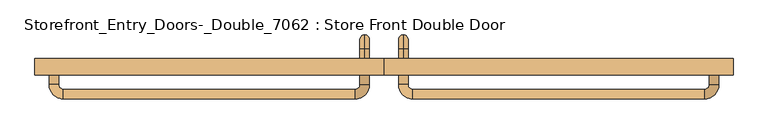
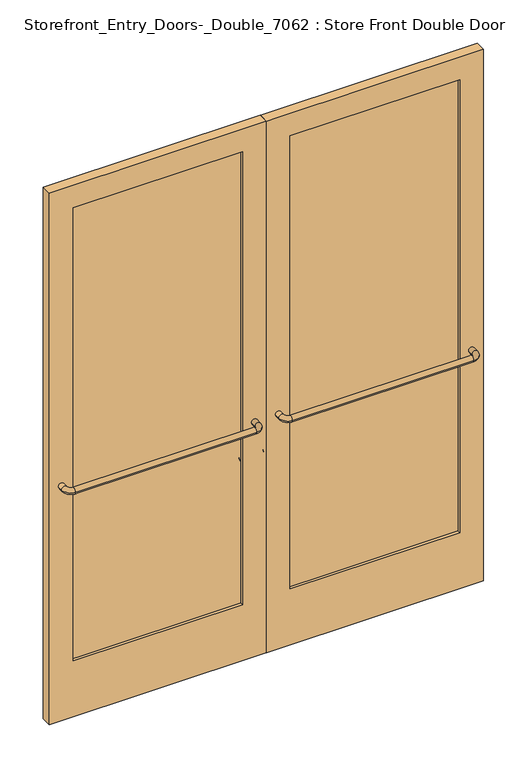
"""IFC4 building model written with IfcOpenShell, lengths in millimetres: door geometry, Storefront_Entry_Doors-_Double_7062 : Store Front Double Door."""

import ifcopenshell
import ifcopenshell.guid

model = None  # the IFC model being written
_history = None  # IfcOwnerHistory: only IFC2X3 demands one
_inside = {}  # id of a spatial element -> (the spatial element, [elements in it])
_under = {}  # id of a project, library or spatial element -> (it, [spatial elements below it])
_declared = {}  # id of a project -> (the project, [libraries it declares])
_typed = {}  # id of a type object -> (the type object, [elements of that type])
_made_of = {}  # id of a material, layer set ... -> (it, [elements and type objects made of it])


def new_model(schema):
    """Start an empty IFC model of exactly this schema.

    Asked for "IFC4X3", IfcOpenShell would pick the latest addendum, in which some entities
    have other attributes; the version numbers below select the first issue.
    IFC2X3 requires an IfcOwnerHistory on every rooted entity: one is made here for all.
    """
    global model, _history
    if schema == "IFC4X3":
        model = ifcopenshell.file(schema_version=(4, 3, 0, 0))
    else:
        model = ifcopenshell.file(schema=schema)
    _inside.clear()
    _under.clear()
    _declared.clear()
    _typed.clear()
    _made_of.clear()
    _history = None
    if model.schema == "IFC2X3":
        org = make("IfcOrganization", Name="unknown")
        user = make(
            "IfcPersonAndOrganization",
            ThePerson=make("IfcPerson", FamilyName="unknown"),
            TheOrganization=org,
        )
        app = make(
            "IfcApplication",
            ApplicationDeveloper=org,
            Version="unknown",
            ApplicationFullName="unknown",
            ApplicationIdentifier="unknown",
        )
        _history = make(
            "IfcOwnerHistory",
            OwningUser=user,
            OwningApplication=app,
            ChangeAction="ADDED",
            CreationDate=0,
        )
    return model


def make(cls, **values):
    """One entity of the class cls with the attributes given. An attribute that is None is left unset."""
    return model.create_entity(
        cls, **{name: value for name, value in values.items() if value is not None}
    )


def rooted(cls, **values):
    """An entity with a GlobalId (a new one), such as an element, a storey or a relation."""
    return make(cls, GlobalId=ifcopenshell.guid.new(), OwnerHistory=_history, **values)


def si_unit(unit_type, name, prefix=None):
    """IfcSIUnit, for example si_unit("LENGTHUNIT", "METRE", prefix="MILLI")."""
    return make("IfcSIUnit", UnitType=unit_type, Prefix=prefix, Name=name)


def assignment(units):
    """IfcUnitAssignment: the units of a project."""
    return None if units is None else make("IfcUnitAssignment", Units=units)


def point(xyz):
    """IfcCartesianPoint."""
    return None if xyz is None else make("IfcCartesianPoint", Coordinates=xyz)


def direction(xyz):
    """IfcDirection."""
    return None if xyz is None else make("IfcDirection", DirectionRatios=xyz)


def frame(location, z_axis=None, x_axis=None):
    """IfcAxis2Placement3D, a coordinate frame: its origin and axes. An axis left out is left unset."""
    return make(
        "IfcAxis2Placement3D",
        Location=point(location),
        Axis=direction(z_axis),
        RefDirection=direction(x_axis),
    )


def origin():
    """The frame at (0, 0, 0) with its axes left unset."""
    return frame((0.0, 0.0, 0.0))


def place(relative_to, where):
    """IfcLocalPlacement: puts the frame where relative to a parent placement (None: the world)."""
    return make(
        "IfcLocalPlacement", PlacementRelTo=relative_to, RelativePlacement=where
    )


def context(
    kind, dimensions, precision=None, world=None, true_north=None, identifier=None
):
    """IfcGeometricRepresentationContext, for example the 3D "Model" context."""
    return make(
        "IfcGeometricRepresentationContext",
        ContextIdentifier=identifier,
        ContextType=kind,
        CoordinateSpaceDimension=dimensions,
        Precision=precision,
        WorldCoordinateSystem=world,
        TrueNorth=true_north,
    )


def project(units=None, contexts=None):
    """IfcProject with its units and contexts."""
    return rooted(
        "IfcProject",
        Name="project",
        RepresentationContexts=contexts,
        UnitsInContext=assignment(units),
    )


def spatial(cls, under=None, at=None, **own):
    """A site, building, storey or space (cls), placed at a placement, below another one or the project."""
    s = rooted(cls, ObjectPlacement=at, **own)
    if under is not None:
        _under.setdefault(under.id(), (under, []))[1].append(s)
    return s


def polyline(points):
    """IfcPolyline through the points."""
    return make("IfcPolyline", Points=[point(p) for p in points])


def circle_curve(where, radius):
    """IfcCircle in the frame where."""
    return make("IfcCircle", Position=where, Radius=radius)


def ellipse_curve(where, semi_axis1, semi_axis2):
    """IfcEllipse in the frame where."""
    return make(
        "IfcEllipse", Position=where, SemiAxis1=semi_axis1, SemiAxis2=semi_axis2
    )


def trimmed(basis, trim1, trim2, sense, master):
    """IfcTrimmedCurve: the piece of a basis curve between two trims."""
    return make(
        "IfcTrimmedCurve",
        BasisCurve=basis,
        Trim1=trim1,
        Trim2=trim2,
        SenseAgreement=sense,
        MasterRepresentation=master,
    )


def outline(outer, holes=None, kind="AREA"):
    """IfcArbitraryClosedProfileDef: a profile drawn as a closed curve; with holes, ...WithVoids."""
    if holes is None:
        return make("IfcArbitraryClosedProfileDef", ProfileType=kind, OuterCurve=outer)
    return make(
        "IfcArbitraryProfileDefWithVoids",
        ProfileType=kind,
        OuterCurve=outer,
        InnerCurves=holes,
    )


def extrude(swept, where, along, depth):
    """IfcExtrudedAreaSolid: the profile swept, set in the frame where, extruded along a direction by depth."""
    return make(
        "IfcExtrudedAreaSolid",
        SweptArea=swept,
        Position=where,
        ExtrudedDirection=direction(along),
        Depth=depth,
    )


def shape(context_of_items, identifier, shape_type, items):
    """IfcShapeRepresentation: the items that make up one representation, for example the "Body"."""
    return make(
        "IfcShapeRepresentation",
        ContextOfItems=context_of_items,
        RepresentationIdentifier=identifier,
        RepresentationType=shape_type,
        Items=items,
    )


def source(mapping_origin, context_of_items, identifier, shape_type, items):
    """IfcRepresentationMap: a shape defined once, which mapped items show again and again."""
    return make(
        "IfcRepresentationMap",
        MappingOrigin=mapping_origin,
        MappedRepresentation=shape(context_of_items, identifier, shape_type, items),
    )


def transform(
    local_origin,
    x_axis=None,
    y_axis=None,
    z_axis=None,
    scale=None,
    scale2=None,
    scale3=None,
    uniform=True,
):
    """IfcCartesianTransformationOperator3D, or its non-uniform kind. x_axis, y_axis, z_axis: its Axis1, 2, 3."""
    if uniform:
        return make(
            "IfcCartesianTransformationOperator3D",
            Axis1=direction(x_axis),
            Axis2=direction(y_axis),
            LocalOrigin=point(local_origin),
            Scale=scale,
            Axis3=direction(z_axis),
        )
    return make(
        "IfcCartesianTransformationOperator3DnonUniform",
        Axis1=direction(x_axis),
        Axis2=direction(y_axis),
        LocalOrigin=point(local_origin),
        Scale=scale,
        Axis3=direction(z_axis),
        Scale2=scale2,
        Scale3=scale3,
    )


def mapped(mapping_source, mapping_target):
    """IfcMappedItem: shows the shape of a source again, moved by a transform."""
    return make(
        "IfcMappedItem", MappingSource=mapping_source, MappingTarget=mapping_target
    )


def made_of(thing, what):
    """Note that an element or type object is made of a material, layer set ...; save() writes the relation."""
    if what is not None:
        _made_of.setdefault(what.id(), (what, []))[1].append(thing)
    return thing


def element(
    cls,
    number,
    at=None,
    inside=None,
    cuts=None,
    type_object=None,
    material=None,
    context=None,
    identifier="Body",
    shape_type=None,
    held_by="IfcProductDefinitionShape",
    body=None,
    shapes=None,
    **own,
):
    """One element of the class cls, such as IfcWall. Its Tag is "e" and its number.

    at: its placement. inside: the storey or other place that contains it. cuts: it is an
    opening in that element (IfcRelVoidsElement). A single representation is given by context,
    identifier, shape_type and body (its items); several are given by shapes. held_by: the class
    of the entity that holds the representations. save() writes the other relations.
    """
    e = rooted(cls, Tag="e%d" % number, ObjectPlacement=at, **own)
    if body is not None:
        shapes = [shape(context, identifier, shape_type, body)]
    if shapes is not None:
        e.Representation = make(held_by, Representations=shapes)
    if inside is not None:
        _inside.setdefault(inside.id(), (inside, []))[1].append(e)
    if cuts is not None:
        rooted(
            "IfcRelVoidsElement", RelatingBuildingElement=cuts, RelatedOpeningElement=e
        )
    if type_object is not None:
        _typed.setdefault(type_object.id(), (type_object, []))[1].append(e)
    return made_of(e, material)


def aggregate(whole, parts):
    """IfcRelAggregates: a whole, such as a stair, and the parts it consists of."""
    return rooted("IfcRelAggregates", RelatingObject=whole, RelatedObjects=parts)


def save(model, path):
    """Write the relations noted so far, then the file.

    IfcRelAggregates (storeys below a building ...), IfcRelContainedInSpatialStructure (elements
    in a storey), IfcRelDefinesByType, IfcRelAssociatesMaterial and IfcRelDeclares: one each for
    every whole, place, type object, material and project.
    """
    for whole, parts in _under.values():
        aggregate(whole, parts)
    for where, things in _inside.values():
        rooted(
            "IfcRelContainedInSpatialStructure",
            RelatedElements=things,
            RelatingStructure=where,
        )
    for kind, things in _typed.values():
        rooted("IfcRelDefinesByType", RelatedObjects=things, RelatingType=kind)
    for what, things in _made_of.values():
        rooted("IfcRelAssociatesMaterial", RelatedObjects=things, RelatingMaterial=what)
    for by, libraries in _declared.values():
        rooted("IfcRelDeclares", RelatingContext=by, RelatedDefinitions=libraries)
    model.write(path)


def plane_surface(at):
    """IfcPlane: the flat surface through the origin of the frame at, square to its z axis."""
    return make("IfcPlane", Position=at)


def cylinder_surface(at, radius):
    """IfcCylindricalSurface: all points at the distance radius from the z axis of the frame at."""
    return make("IfcCylindricalSurface", Position=at, Radius=radius)


def revolved_surface(curve, axis_point, axis_direction):
    """IfcSurfaceOfRevolution: the curve turned about the line through axis_point along axis_direction."""
    return make(
        "IfcSurfaceOfRevolution",
        SweptCurve=make("IfcArbitraryOpenProfileDef", ProfileType="CURVE", Curve=curve),
        AxisPosition=make("IfcAxis1Placement", Location=point(axis_point), Axis=direction(axis_direction)),
    )


def advanced_brep(points, edges, surfaces, faces):
    """IfcAdvancedBrep: a solid bounded by faces that lie on surfaces and meet in shared edges.

    An edge is (start, end): straight between two places in points (the first is 0);
    or (start, end, curve); or (start, end, curve, False) where it runs against its curve.
    A face is (place in surfaces, loops), or (place, loops, False) where it looks against
    its surface's normal. A loop lists edges by number (the first is 1), with a minus sign
    where the edge is run from its end to its start. The first loop is the outer one.
    """
    corners = [point(p) for p in points]
    vertices = [make("IfcVertexPoint", VertexGeometry=c) for c in corners]
    made = []
    for start, end, *more in edges:
        made.append(
            make(
                "IfcEdgeCurve",
                EdgeStart=vertices[start],
                EdgeEnd=vertices[end],
                EdgeGeometry=more[0] if more else make("IfcPolyline", Points=[corners[start], corners[end]]),
                SameSense=more[1] if len(more) > 1 else True,
            )
        )
    hull = []
    for where, loops, *sense in faces:
        bounds = []
        for j, loop in enumerate(loops):
            ring = [make("IfcOrientedEdge", EdgeElement=made[abs(k) - 1], Orientation=k > 0) for k in loop]
            bounds.append(
                make(
                    "IfcFaceOuterBound" if j == 0 else "IfcFaceBound",
                    Bound=make("IfcEdgeLoop", EdgeList=ring),
                    Orientation=True,
                )
            )
        hull.append(make("IfcAdvancedFace", Bounds=bounds, FaceSurface=surfaces[where], SameSense=sense[0] if sense else True))
    return make("IfcAdvancedBrep", Outer=make("IfcClosedShell", CfsFaces=hull))


def storefront_entry_doors_double_7062_store_front_double_door_b38478ba(model_context):
    return source(origin(), model_context, "Body", "SolidModel", [
        advanced_brep(
        [(51.59375, 50.8, 1079.5), (51.59375, 50.8, 1054.1), (51.59375, 76.2, 1079.5), (51.59375, 76.2, 1054.1), (51.59375, 88.9, 1041.4), (51.59375, 114.3, 1041.4), (51.59375, 114.3, 863.6), (51.59375, 88.9, 863.6), (51.59375, 76.2, 850.9), (51.59375, 76.2, 825.5), (51.59375, 50.8, 825.5), (51.59375, 50.8, 850.9)],
        [
            (0, 1, circle_curve(frame((51.59375, 50.8, 1066.8), z_axis=(0.0, -1.0, 0.0), x_axis=(0.0, 0.0, -1.0)), 12.7)),
            (1, 0, circle_curve(frame((51.59375, 50.8, 1066.8), z_axis=(0.0, -1.0, 0.0), x_axis=(0.0, 0.0, -1.0)), 12.7)),
            (0, 2),
            (2, 3, circle_curve(frame((51.59375, 76.2, 1066.8), z_axis=(0.0, -1.0, 0.0), x_axis=(0.0, 0.0, -1.0)), 12.7)),
            (3, 1),
            (3, 2, circle_curve(frame((51.59375, 76.2, 1066.8), z_axis=(0.0, -1.0, 0.0), x_axis=(0.0, 0.0, -1.0)), 12.7)),
            (4, 3, circle_curve(frame((51.59375, 76.2, 1041.4), z_axis=(1.0, 0.0, 0.0), x_axis=(0.0, 0.0, 1.0)), 12.7)),
            (2, 5, circle_curve(frame((51.59375, 76.2, 1041.4), z_axis=(-1.0, 0.0, 0.0), x_axis=(0.0, 0.0, 1.0)), 38.1)),
            (5, 4, circle_curve(frame((51.59375, 101.6, 1041.4), z_axis=(0.0, 0.0, 1.0), x_axis=(0.0, -1.0, 0.0)), 12.7)),
            (4, 5, circle_curve(frame((51.59375, 101.6, 1041.4), z_axis=(0.0, 0.0, 1.0), x_axis=(0.0, -1.0, 0.0)), 12.7)),
            (5, 6),
            (6, 7, circle_curve(frame((51.59375, 101.6, 863.6), z_axis=(0.0, 0.0, 1.0), x_axis=(0.0, -1.0, 0.0)), 12.7)),
            (7, 4),
            (7, 6, circle_curve(frame((51.59375, 101.6, 863.6), z_axis=(0.0, 0.0, 1.0), x_axis=(0.0, -1.0, 0.0)), 12.7)),
            (8, 7, circle_curve(frame((51.59375, 76.2, 863.6), z_axis=(1.0, 0.0, 0.0), x_axis=(0.0, 1.0, 0.0)), 12.7)),
            (6, 9, circle_curve(frame((51.59375, 76.2, 863.6), z_axis=(-1.0, 0.0, 0.0), x_axis=(0.0, 1.0, 0.0)), 38.1)),
            (9, 8, circle_curve(frame((51.59375, 76.2, 838.2), z_axis=(0.0, 1.0, 0.0), x_axis=(0.0, 0.0, 1.0)), 12.7)),
            (8, 9, circle_curve(frame((51.59375, 76.2, 838.2), z_axis=(0.0, 1.0, 0.0), x_axis=(0.0, 0.0, 1.0)), 12.7)),
            (10, 11, circle_curve(frame((51.59375, 50.8, 838.2), z_axis=(0.0, -1.0, 0.0), x_axis=(0.0, 0.0, 1.0)), 12.7)),
            (11, 10, circle_curve(frame((51.59375, 50.8, 838.2), z_axis=(0.0, -1.0, 0.0), x_axis=(0.0, 0.0, 1.0)), 12.7)),
            (9, 10),
            (11, 8),
        ],
        [
            plane_surface(frame((51.59375, 50.8, 1066.8), z_axis=(0.0, -1.0, 0.0), x_axis=(-1.0, 0.0, 0.0))),
            cylinder_surface(frame((51.59375, 50.8, 1066.8), z_axis=(0.0, -1.0, 0.0), x_axis=(0.0, 0.0, -1.0)), 12.7),
            revolved_surface(trimmed(ellipse_curve(frame((51.59375, 76.2, 1066.8), z_axis=(0.0, -1.0, 0.0), x_axis=(0.0, 0.0, -1.0)), 12.7, 12.7), [point((51.59375, 76.2, 1079.5))], [point((51.59375, 76.2, 1054.1))], True, "CARTESIAN"), (51.59375, 76.2, 1041.4), (-1.0, 0.0, 0.0)),
            revolved_surface(trimmed(ellipse_curve(frame((51.59375, 76.2, 1066.8), z_axis=(0.0, -1.0, 0.0), x_axis=(0.0, 0.0, -1.0)), 12.7, 12.7), [point((51.59375, 76.2, 1054.1))], [point((51.59375, 76.2, 1079.5))], True, "CARTESIAN"), (51.59375, 76.2, 1041.4), (-1.0, 0.0, 0.0)),
            cylinder_surface(frame((51.59375, 101.6, 1041.4), z_axis=(0.0, 0.0, 1.0), x_axis=(0.0, -1.0, 0.0)), 12.7),
            revolved_surface(trimmed(ellipse_curve(frame((51.59375, 101.6, 863.6), z_axis=(0.0, 0.0, 1.0), x_axis=(0.0, -1.0, 0.0)), 12.7, 12.7), [point((51.59375, 114.3, 863.6))], [point((51.59375, 88.9, 863.6))], True, "CARTESIAN"), (51.59375, 76.2, 863.6), (-1.0, 0.0, 0.0)),
            revolved_surface(trimmed(ellipse_curve(frame((51.59375, 101.6, 863.6), z_axis=(0.0, 0.0, 1.0), x_axis=(0.0, -1.0, 0.0)), 12.7, 12.7), [point((51.59375, 88.9, 863.6))], [point((51.59375, 114.3, 863.6))], True, "CARTESIAN"), (51.59375, 76.2, 863.6), (-1.0, 0.0, 0.0)),
            plane_surface(frame((51.59375, 50.8, 838.2), z_axis=(0.0, -1.0, 0.0), x_axis=(-1.0, 0.0, 0.0))),
            cylinder_surface(frame((51.59375, 76.2, 838.2), z_axis=(0.0, 1.0, 0.0), x_axis=(0.0, 0.0, 1.0)), 12.7),
        ],
        [
            (0, [[1, 2]]),
            (1, [[-1, 3, 4, 5]]),
            (1, [[-2, -5, 6, -3]]),
            (2, [[7, -4, 8, 9]]),
            (3, [[-8, -6, -7, 10]]),
            (4, [[-9, 11, 12, 13]]),
            (4, [[-10, -13, 14, -11]]),
            (5, [[15, -12, 16, 17]]),
            (6, [[-16, -14, -15, 18]]),
            (7, [[19, 20]]),
            (8, [[-17, 21, -20, 22]]),
            (8, [[-18, -22, -19, -21]]),
        ],
    ),
        advanced_brep(
        [(869.0428571, 6.35, 1066.8), (894.4428571, 6.35, 1066.8), (869.0428571, -19.05, 1066.8), (894.4428571, -19.05, 1066.8), (856.3428571, -57.15, 1066.8), (856.3428571, -31.75, 1066.8), (76.99375, -31.75, 1066.8), (76.99375, -57.15, 1066.8), (38.89375, -19.05, 1066.8), (64.29375, -19.05, 1066.8), (64.29375, 6.35, 1066.8), (38.89375, 6.35, 1066.8)],
        [
            (0, 1, circle_curve(frame((881.7428571, 6.35, 1066.8), z_axis=(0.0, 1.0, 0.0), x_axis=(1.0, 0.0, 0.0)), 12.7)),
            (1, 0, circle_curve(frame((881.7428571, 6.35, 1066.8), z_axis=(0.0, 1.0, 0.0), x_axis=(1.0, 0.0, 0.0)), 12.7)),
            (0, 2),
            (2, 3, circle_curve(frame((881.7428571, -19.05, 1066.8), z_axis=(0.0, 1.0, 0.0), x_axis=(1.0, 0.0, 0.0)), 12.7)),
            (3, 1),
            (3, 2, circle_curve(frame((881.7428571, -19.05, 1066.8), z_axis=(0.0, 1.0, 0.0), x_axis=(1.0, 0.0, 0.0)), 12.7)),
            (4, 3, circle_curve(frame((856.3428571, -19.05, 1066.8), z_axis=(0.0, 0.0, 1.0), x_axis=(1.0, 0.0, 0.0)), 38.1)),
            (2, 5, circle_curve(frame((856.3428571, -19.05, 1066.8), z_axis=(0.0, 0.0, -1.0), x_axis=(1.0, 0.0, 0.0)), 12.7)),
            (5, 4, circle_curve(frame((856.3428571, -44.45, 1066.8), z_axis=(1.0, 0.0, 0.0), x_axis=(0.0, -1.0, 0.0)), 12.7)),
            (4, 5, circle_curve(frame((856.3428571, -44.45, 1066.8), z_axis=(1.0, 0.0, 0.0), x_axis=(0.0, -1.0, 0.0)), 12.7)),
            (5, 6),
            (6, 7, circle_curve(frame((76.99375, -44.45, 1066.8), z_axis=(1.0, 0.0, 0.0), x_axis=(0.0, -1.0, 0.0)), 12.7)),
            (7, 4),
            (7, 6, circle_curve(frame((76.99375, -44.45, 1066.8), z_axis=(1.0, 0.0, 0.0), x_axis=(0.0, -1.0, 0.0)), 12.7)),
            (8, 7, circle_curve(frame((76.99375, -19.05, 1066.8), z_axis=(0.0, 0.0, 1.0), x_axis=(0.0, -1.0, 0.0)), 38.1)),
            (6, 9, circle_curve(frame((76.99375, -19.05, 1066.8), z_axis=(0.0, 0.0, -1.0), x_axis=(0.0, -1.0, 0.0)), 12.7)),
            (9, 8, circle_curve(frame((51.59375, -19.05, 1066.8), z_axis=(0.0, -1.0, 0.0), x_axis=(-1.0, 0.0, 0.0)), 12.7)),
            (8, 9, circle_curve(frame((51.59375, -19.05, 1066.8), z_axis=(0.0, -1.0, 0.0), x_axis=(-1.0, 0.0, 0.0)), 12.7)),
            (10, 11, circle_curve(frame((51.59375, 6.35, 1066.8), z_axis=(0.0, 1.0, 0.0), x_axis=(-1.0, 0.0, 0.0)), 12.7)),
            (11, 10, circle_curve(frame((51.59375, 6.35, 1066.8), z_axis=(0.0, 1.0, 0.0), x_axis=(-1.0, 0.0, 0.0)), 12.7)),
            (9, 10),
            (11, 8),
        ],
        [
            plane_surface(frame((881.7428571, 6.35, 1066.8), z_axis=(0.0, 1.0, 0.0), x_axis=(0.0, 0.0, 1.0))),
            cylinder_surface(frame((881.7428571, 6.35, 1066.8), z_axis=(0.0, 1.0, 0.0), x_axis=(1.0, 0.0, 0.0)), 12.7),
            revolved_surface(trimmed(ellipse_curve(frame((881.7428571, -19.05, 1066.8), z_axis=(0.0, 1.0, 0.0), x_axis=(1.0, 0.0, 0.0)), 12.7, 12.7), [point((869.0428571, -19.05, 1066.8))], [point((894.4428571, -19.05, 1066.8))], True, "CARTESIAN"), (856.3428571, -19.05, 1066.8), (0.0, 0.0, -1.0)),
            revolved_surface(trimmed(ellipse_curve(frame((881.7428571, -19.05, 1066.8), z_axis=(0.0, 1.0, 0.0), x_axis=(1.0, 0.0, 0.0)), 12.7, 12.7), [point((894.4428571, -19.05, 1066.8))], [point((869.0428571, -19.05, 1066.8))], True, "CARTESIAN"), (856.3428571, -19.05, 1066.8), (0.0, 0.0, -1.0)),
            cylinder_surface(frame((856.3428571, -44.45, 1066.8), z_axis=(1.0, 0.0, 0.0), x_axis=(0.0, -1.0, 0.0)), 12.7),
            revolved_surface(trimmed(ellipse_curve(frame((76.99375, -44.45, 1066.8), z_axis=(1.0, 0.0, 0.0), x_axis=(0.0, -1.0, 0.0)), 12.7, 12.7), [point((76.99375, -31.75, 1066.8))], [point((76.99375, -57.15, 1066.8))], True, "CARTESIAN"), (76.99375, -19.05, 1066.8), (0.0, 0.0, -1.0)),
            revolved_surface(trimmed(ellipse_curve(frame((76.99375, -44.45, 1066.8), z_axis=(1.0, 0.0, 0.0), x_axis=(0.0, -1.0, 0.0)), 12.7, 12.7), [point((76.99375, -57.15, 1066.8))], [point((76.99375, -31.75, 1066.8))], True, "CARTESIAN"), (76.99375, -19.05, 1066.8), (0.0, 0.0, -1.0)),
            plane_surface(frame((51.59375, 6.35, 1066.8), z_axis=(0.0, 1.0, 0.0), x_axis=(0.0, 0.0, 1.0))),
            cylinder_surface(frame((51.59375, -19.05, 1066.8), z_axis=(0.0, -1.0, 0.0), x_axis=(-1.0, 0.0, 0.0)), 12.7),
        ],
        [
            (0, [[1, 2]]),
            (1, [[-1, 3, 4, 5]]),
            (1, [[-2, -5, 6, -3]]),
            (2, [[7, -4, 8, 9]]),
            (3, [[-8, -6, -7, 10]]),
            (4, [[-9, 11, 12, 13]]),
            (4, [[-10, -13, 14, -11]]),
            (5, [[15, -12, 16, 17]]),
            (6, [[-16, -14, -15, 18]]),
            (7, [[19, 20]]),
            (8, [[-17, 21, -20, 22]]),
            (8, [[-18, -22, -19, -21]]),
        ],
    ),
        advanced_brep(
        [(-51.59375, 50.8, 1054.1), (-51.59375, 50.8, 1079.5), (-51.59375, 76.2, 1054.1), (-51.59375, 76.2, 1079.5), (-51.59375, 114.3, 1041.4), (-51.59375, 88.9, 1041.4), (-51.59375, 88.9, 863.6), (-51.59375, 114.3, 863.6), (-51.59375, 76.2, 825.5), (-51.59375, 76.2, 850.9), (-51.59375, 50.8, 850.9), (-51.59375, 50.8, 825.5)],
        [
            (0, 1, circle_curve(frame((-51.59375, 50.8, 1066.8), z_axis=(0.0, -1.0, 0.0), x_axis=(0.0, 0.0, 1.0)), 12.7)),
            (1, 0, circle_curve(frame((-51.59375, 50.8, 1066.8), z_axis=(0.0, -1.0, 0.0), x_axis=(0.0, 0.0, 1.0)), 12.7)),
            (0, 2),
            (2, 3, circle_curve(frame((-51.59375, 76.2, 1066.8), z_axis=(0.0, -1.0, 0.0), x_axis=(0.0, 0.0, 1.0)), 12.7)),
            (3, 1),
            (3, 2, circle_curve(frame((-51.59375, 76.2, 1066.8), z_axis=(0.0, -1.0, 0.0), x_axis=(0.0, 0.0, 1.0)), 12.7)),
            (4, 3, circle_curve(frame((-51.59375, 76.2, 1041.4), z_axis=(1.0, 0.0, 0.0), x_axis=(0.0, 0.0, 1.0)), 38.1)),
            (2, 5, circle_curve(frame((-51.59375, 76.2, 1041.4), z_axis=(-1.0, 0.0, 0.0), x_axis=(0.0, 0.0, 1.0)), 12.7)),
            (5, 4, circle_curve(frame((-51.59375, 101.6, 1041.4), z_axis=(0.0, 0.0, 1.0), x_axis=(0.0, 1.0, 0.0)), 12.7)),
            (4, 5, circle_curve(frame((-51.59375, 101.6, 1041.4), z_axis=(0.0, 0.0, 1.0), x_axis=(0.0, 1.0, 0.0)), 12.7)),
            (5, 6),
            (6, 7, circle_curve(frame((-51.59375, 101.6, 863.6), z_axis=(0.0, 0.0, 1.0), x_axis=(0.0, 1.0, 0.0)), 12.7)),
            (7, 4),
            (7, 6, circle_curve(frame((-51.59375, 101.6, 863.6), z_axis=(0.0, 0.0, 1.0), x_axis=(0.0, 1.0, 0.0)), 12.7)),
            (8, 7, circle_curve(frame((-51.59375, 76.2, 863.6), z_axis=(1.0, 0.0, 0.0), x_axis=(0.0, 1.0, 0.0)), 38.1)),
            (6, 9, circle_curve(frame((-51.59375, 76.2, 863.6), z_axis=(-1.0, 0.0, 0.0), x_axis=(0.0, 1.0, 0.0)), 12.7)),
            (9, 8, circle_curve(frame((-51.59375, 76.2, 838.2), z_axis=(0.0, 1.0, 0.0), x_axis=(0.0, 0.0, -1.0)), 12.7)),
            (8, 9, circle_curve(frame((-51.59375, 76.2, 838.2), z_axis=(0.0, 1.0, 0.0), x_axis=(0.0, 0.0, -1.0)), 12.7)),
            (10, 11, circle_curve(frame((-51.59375, 50.8, 838.2), z_axis=(0.0, -1.0, 0.0), x_axis=(0.0, 0.0, -1.0)), 12.7)),
            (11, 10, circle_curve(frame((-51.59375, 50.8, 838.2), z_axis=(0.0, -1.0, 0.0), x_axis=(0.0, 0.0, -1.0)), 12.7)),
            (9, 10),
            (11, 8),
        ],
        [
            plane_surface(frame((-51.59375, 50.8, 1066.8), z_axis=(0.0, -1.0, 0.0), x_axis=(1.0, 0.0, 0.0))),
            cylinder_surface(frame((-51.59375, 50.8, 1066.8), z_axis=(0.0, -1.0, 0.0), x_axis=(0.0, 0.0, 1.0)), 12.7),
            revolved_surface(trimmed(ellipse_curve(frame((-51.59375, 76.2, 1066.8), z_axis=(0.0, -1.0, 0.0), x_axis=(0.0, 0.0, 1.0)), 12.7, 12.7), [point((-51.59375, 76.2, 1054.1))], [point((-51.59375, 76.2, 1079.5))], True, "CARTESIAN"), (-51.59375, 76.2, 1041.4), (-1.0, 0.0, 0.0)),
            revolved_surface(trimmed(ellipse_curve(frame((-51.59375, 76.2, 1066.8), z_axis=(0.0, -1.0, 0.0), x_axis=(0.0, 0.0, 1.0)), 12.7, 12.7), [point((-51.59375, 76.2, 1079.5))], [point((-51.59375, 76.2, 1054.1))], True, "CARTESIAN"), (-51.59375, 76.2, 1041.4), (-1.0, 0.0, 0.0)),
            cylinder_surface(frame((-51.59375, 101.6, 1041.4), z_axis=(0.0, 0.0, 1.0), x_axis=(0.0, 1.0, 0.0)), 12.7),
            revolved_surface(trimmed(ellipse_curve(frame((-51.59375, 101.6, 863.6), z_axis=(0.0, 0.0, 1.0), x_axis=(0.0, 1.0, 0.0)), 12.7, 12.7), [point((-51.59375, 88.9, 863.6))], [point((-51.59375, 114.3, 863.6))], True, "CARTESIAN"), (-51.59375, 76.2, 863.6), (-1.0, 0.0, 0.0)),
            revolved_surface(trimmed(ellipse_curve(frame((-51.59375, 101.6, 863.6), z_axis=(0.0, 0.0, 1.0), x_axis=(0.0, 1.0, 0.0)), 12.7, 12.7), [point((-51.59375, 114.3, 863.6))], [point((-51.59375, 88.9, 863.6))], True, "CARTESIAN"), (-51.59375, 76.2, 863.6), (-1.0, 0.0, 0.0)),
            plane_surface(frame((-51.59375, 50.8, 838.2), z_axis=(0.0, -1.0, 0.0), x_axis=(1.0, 0.0, 0.0))),
            cylinder_surface(frame((-51.59375, 76.2, 838.2), z_axis=(0.0, 1.0, 0.0), x_axis=(0.0, 0.0, -1.0)), 12.7),
        ],
        [
            (0, [[1, 2]]),
            (1, [[-1, 3, 4, 5]]),
            (1, [[-2, -5, 6, -3]]),
            (2, [[7, -4, 8, 9]]),
            (3, [[-8, -6, -7, 10]]),
            (4, [[-9, 11, 12, 13]]),
            (4, [[-10, -13, 14, -11]]),
            (5, [[15, -12, 16, 17]]),
            (6, [[-16, -14, -15, 18]]),
            (7, [[19, 20]]),
            (8, [[-17, 21, -20, 22]]),
            (8, [[-18, -22, -19, -21]]),
        ],
    ),
        advanced_brep(
        [(-64.29375, 6.35, 1066.8), (-38.89375, 6.35, 1066.8), (-64.29375, -19.05, 1066.8), (-38.89375, -19.05, 1066.8), (-76.99375, -57.15, 1066.8), (-76.99375, -31.75, 1066.8), (-856.3428571, -31.75, 1066.8), (-856.3428571, -57.15, 1066.8), (-894.4428571, -19.05, 1066.8), (-869.0428571, -19.05, 1066.8), (-869.0428571, 6.35, 1066.8), (-894.4428571, 6.35, 1066.8)],
        [
            (0, 1, circle_curve(frame((-51.59375, 6.35, 1066.8), z_axis=(0.0, 1.0, 0.0), x_axis=(1.0, 0.0, 0.0)), 12.7)),
            (1, 0, circle_curve(frame((-51.59375, 6.35, 1066.8), z_axis=(0.0, 1.0, 0.0), x_axis=(1.0, 0.0, 0.0)), 12.7)),
            (0, 2),
            (2, 3, circle_curve(frame((-51.59375, -19.05, 1066.8), z_axis=(0.0, 1.0, 0.0), x_axis=(1.0, 0.0, 0.0)), 12.7)),
            (3, 1),
            (3, 2, circle_curve(frame((-51.59375, -19.05, 1066.8), z_axis=(0.0, 1.0, 0.0), x_axis=(1.0, 0.0, 0.0)), 12.7)),
            (4, 3, circle_curve(frame((-76.99375, -19.05, 1066.8), z_axis=(0.0, 0.0, 1.0), x_axis=(1.0, 0.0, 0.0)), 38.1)),
            (2, 5, circle_curve(frame((-76.99375, -19.05, 1066.8), z_axis=(0.0, 0.0, -1.0), x_axis=(1.0, 0.0, 0.0)), 12.7)),
            (5, 4, circle_curve(frame((-76.99375, -44.45, 1066.8), z_axis=(1.0, 0.0, 0.0), x_axis=(0.0, -1.0, 0.0)), 12.7)),
            (4, 5, circle_curve(frame((-76.99375, -44.45, 1066.8), z_axis=(1.0, 0.0, 0.0), x_axis=(0.0, -1.0, 0.0)), 12.7)),
            (5, 6),
            (6, 7, circle_curve(frame((-856.3428571, -44.45, 1066.8), z_axis=(1.0, 0.0, 0.0), x_axis=(0.0, -1.0, 0.0)), 12.7)),
            (7, 4),
            (7, 6, circle_curve(frame((-856.3428571, -44.45, 1066.8), z_axis=(1.0, 0.0, 0.0), x_axis=(0.0, -1.0, 0.0)), 12.7)),
            (8, 7, circle_curve(frame((-856.3428571, -19.05, 1066.8), z_axis=(0.0, 0.0, 1.0), x_axis=(0.0, -1.0, 0.0)), 38.1)),
            (6, 9, circle_curve(frame((-856.3428571, -19.05, 1066.8), z_axis=(0.0, 0.0, -1.0), x_axis=(0.0, -1.0, 0.0)), 12.7)),
            (9, 8, circle_curve(frame((-881.7428571, -19.05, 1066.8), z_axis=(0.0, -1.0, 0.0), x_axis=(-1.0, 0.0, 0.0)), 12.7)),
            (8, 9, circle_curve(frame((-881.7428571, -19.05, 1066.8), z_axis=(0.0, -1.0, 0.0), x_axis=(-1.0, 0.0, 0.0)), 12.7)),
            (10, 11, circle_curve(frame((-881.7428571, 6.35, 1066.8), z_axis=(0.0, 1.0, 0.0), x_axis=(-1.0, 0.0, 0.0)), 12.7)),
            (11, 10, circle_curve(frame((-881.7428571, 6.35, 1066.8), z_axis=(0.0, 1.0, 0.0), x_axis=(-1.0, 0.0, 0.0)), 12.7)),
            (9, 10),
            (11, 8),
        ],
        [
            plane_surface(frame((-51.59375, 6.35, 1066.8), z_axis=(0.0, 1.0, 0.0), x_axis=(0.0, 0.0, 1.0))),
            cylinder_surface(frame((-51.59375, 6.35, 1066.8), z_axis=(0.0, 1.0, 0.0), x_axis=(1.0, 0.0, 0.0)), 12.7),
            revolved_surface(trimmed(ellipse_curve(frame((-51.59375, -19.05, 1066.8), z_axis=(0.0, 1.0, 0.0), x_axis=(1.0, 0.0, 0.0)), 12.7, 12.7), [point((-64.29375, -19.05, 1066.8))], [point((-38.89375, -19.05, 1066.8))], True, "CARTESIAN"), (-76.99375, -19.05, 1066.8), (0.0, 0.0, -1.0)),
            revolved_surface(trimmed(ellipse_curve(frame((-51.59375, -19.05, 1066.8), z_axis=(0.0, 1.0, 0.0), x_axis=(1.0, 0.0, 0.0)), 12.7, 12.7), [point((-38.89375, -19.05, 1066.8))], [point((-64.29375, -19.05, 1066.8))], True, "CARTESIAN"), (-76.99375, -19.05, 1066.8), (0.0, 0.0, -1.0)),
            cylinder_surface(frame((-76.99375, -44.45, 1066.8), z_axis=(1.0, 0.0, 0.0), x_axis=(0.0, -1.0, 0.0)), 12.7),
            revolved_surface(trimmed(ellipse_curve(frame((-856.3428571, -44.45, 1066.8), z_axis=(1.0, 0.0, 0.0), x_axis=(0.0, -1.0, 0.0)), 12.7, 12.7), [point((-856.3428571, -31.75, 1066.8))], [point((-856.3428571, -57.15, 1066.8))], True, "CARTESIAN"), (-856.3428571, -19.05, 1066.8), (0.0, 0.0, -1.0)),
            revolved_surface(trimmed(ellipse_curve(frame((-856.3428571, -44.45, 1066.8), z_axis=(1.0, 0.0, 0.0), x_axis=(0.0, -1.0, 0.0)), 12.7, 12.7), [point((-856.3428571, -57.15, 1066.8))], [point((-856.3428571, -31.75, 1066.8))], True, "CARTESIAN"), (-856.3428571, -19.05, 1066.8), (0.0, 0.0, -1.0)),
            plane_surface(frame((-881.7428571, 6.35, 1066.8), z_axis=(0.0, 1.0, 0.0), x_axis=(0.0, 0.0, 1.0))),
            cylinder_surface(frame((-881.7428571, -19.05, 1066.8), z_axis=(0.0, -1.0, 0.0), x_axis=(-1.0, 0.0, 0.0)), 12.7),
        ],
        [
            (0, [[1, 2]]),
            (1, [[-1, 3, 4, 5]]),
            (1, [[-2, -5, 6, -3]]),
            (2, [[7, -4, 8, 9]]),
            (3, [[-8, -6, -7, 10]]),
            (4, [[-9, 11, 12, 13]]),
            (4, [[-10, -13, 14, -11]]),
            (5, [[15, -12, 16, 17]]),
            (6, [[-16, -14, -15, 18]]),
            (7, [[19, 20]]),
            (8, [[-17, 21, -20, 22]]),
            (8, [[-18, -22, -19, -21]]),
        ],
    ),
        extrude(outline(polyline([(830.9428571, 19.05), (102.39375, 19.05), (102.39375, 38.1), (830.9428571, 38.1), (830.9428571, 19.05)])), frame((0.0, 0.0, 254.0), z_axis=(0.0, 0.0, 1.0), x_axis=(1.0, 0.0, 0.0)), (0.0, 0.0, 1.0), 2057.4),
        extrude(outline(polyline([(-102.39375, 19.05), (-830.9428571, 19.05), (-830.9428571, 38.1), (-102.39375, 38.1), (-102.39375, 19.05)])), frame((0.0, 0.0, 254.0), z_axis=(0.0, 0.0, 1.0), x_axis=(1.0, 0.0, 0.0)), (0.0, 0.0, 1.0), 2057.4),
        extrude(outline(polyline([(2413.0, 0.79375), (0.0, 0.79375), (0.0, 932.5428571), (2413.0, 932.5428571), (2413.0, 0.79375)]), holes=[polyline([(2311.4, 102.39375), (2311.4, 830.9428571), (254.0, 830.9428571), (254.0, 102.39375), (2311.4, 102.39375)])]), frame((0.0, 6.35, 0.0), z_axis=(0.0, 1.0, 0.0), x_axis=(0.0, 0.0, 1.0)), (0.0, 0.0, 1.0), 44.45),
        extrude(outline(polyline([(2413.0, -0.79375), (2413.0, -932.5428571), (0.0, -932.5428571), (0.0, -0.79375), (2413.0, -0.79375)]), holes=[polyline([(2311.4, -830.9428571), (2311.4, -102.39375), (254.0, -102.39375), (254.0, -830.9428571), (2311.4, -830.9428571)])]), frame((0.0, 6.35, 0.0), z_axis=(0.0, 1.0, 0.0), x_axis=(0.0, 0.0, 1.0)), (0.0, 0.0, 1.0), 44.45),
    ])


if __name__ == "__main__":
    model = new_model("IFC4")
    model_context = context("Model", 3, world=origin())
    ifc_project = project(units=[si_unit("LENGTHUNIT", "METRE", prefix="MILLI")], contexts=[model_context])
    site = spatial("IfcSite", under=ifc_project)
    building = spatial("IfcBuilding", under=site)
    placement = place(None, origin())
    storefront_entry_doors_double_7062_store_front_double_door_shape = storefront_entry_doors_double_7062_store_front_double_door_b38478ba(model_context)
    element("IfcDoor", 1, ObjectType="Storefront_Entry_Doors-_Double_7062 : Store Front Double Door", at=placement, inside=building, context=model_context, shape_type="MappedRepresentation", body=[
        mapped(storefront_entry_doors_double_7062_store_front_double_door_shape, transform((0.0, 0.0, 0.0), x_axis=(1.0, 0.0, 0.0), y_axis=(0.0, 1.0, 0.0), z_axis=(0.0, 0.0, 1.0))),
    ])
    save(model, "model.ifc")

# Revit data of these elements
# Type "Storefront_Entry_Doors-_Double_7062 : Store Front Double Door"
#   Type Mark = "20"
#   Assembly Code = "B2030110"
#   Top Rail = 0.333333 ft
#   Side Rail = 0.333333 ft
#   Rail Height AFF = 3.5 ft
#   Offset = 0.166667 ft
#   Bottom Rail Width = 0.833333 ft
#   Material = Metal - Aluminum
#   Glazing Material = Glass
#   Function = (empty or 0)
# Element 1 (IfcDoor, "Storefront_Entry_Doors-_Double_7062 : Store Front Double Door")
#   Materials on its faces: "Metal - Aluminum", "Glass"
# Materials
#   "Metal - Aluminum": class "Metal", colour RGB 247 247 247, transparency 0
#   "Glass": class "Glass", colour RGB 218 227 224, transparency 0.85, Description = "Soda Lime Glass", Cost = 0
